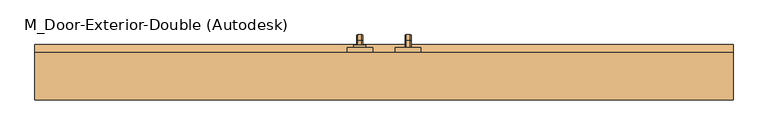
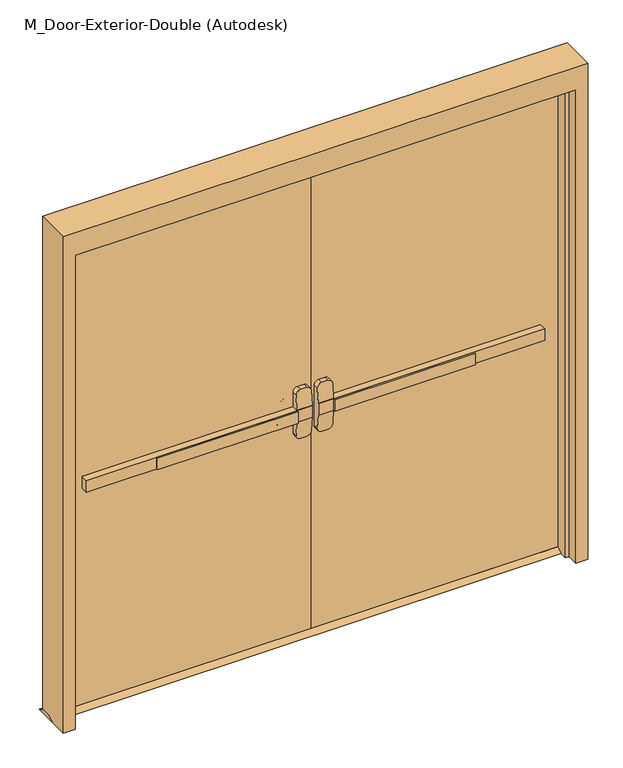
"""IFC4 building model written with IfcOpenShell, lengths in millimetres: door geometry, M_Door-Exterior-Double (Autodesk) : H_DR_AMD_Double Door_Ext_Steel_2100x2100_Panic Bar."""

from ifc_helpers import new_model, si_unit, point, frame, frame_2d, origin, place, context, project, spatial, polyline, circle_curve, ellipse_curve, trimmed, segment, composite_curve, outline, extrude, faceted_brep, source, transform, mapped, element, save
from ifc_brep_helpers import plane_surface, cylinder_surface, revolved_surface, advanced_brep


def m_door_exterior_double_autodesk_2b3cb0e1(model_context):
    return source(origin(), model_context, "Body", "SolidModel", [
        extrude(outline(polyline([(-666.1333333, -41.75), (-666.1333333, -35.4), (-76.2, -35.4), (-76.2, -41.75), (-666.1333333, -41.75)])), frame((0.0, 0.0, 974.6), z_axis=(0.0, 0.0, 1.0), x_axis=(1.0, 0.0, 0.0)), (0.0, 0.0, 1.0), 50.8),
        advanced_brep(
        [(-12.7, -35.4, 1025.4), (-76.2, -35.4, 1025.4), (-961.1, -35.4, 1025.4), (-961.1, -35.4, 974.6), (-76.2, -35.4, 974.6), (-12.7, -35.4, 974.6), (-961.1, -3.65, 1025.4), (-76.2, -3.65, 1025.4), (-76.2, -3.65, 1088.9), (-57.15, -3.65, 1107.95), (-31.75, -3.65, 1107.95), (-12.7, -3.65, 1088.9), (-12.7, -3.65, 911.1), (-31.75, -3.65, 892.05), (-57.15, -3.65, 892.05), (-76.2, -3.65, 911.1), (-76.2, -3.65, 974.6), (-961.1, -3.65, 974.6), (-12.7, -32.2247533, 1025.4), (-76.2, -32.2247533, 1025.4), (-12.7, -32.2247533, 974.6), (-12.7, -27.2145731, 911.1), (-12.7, -27.2145731, 1088.9), (-76.2, -32.2247533, 974.6), (-76.2, -27.2145731, 1088.9), (-76.2, -27.2145731, 911.1), (-57.15, -25.711519, 1107.95), (-31.75, -25.711519, 1107.95), (-31.75, -25.711519, 892.05), (-57.15, -25.711519, 892.05)],
        [
            (0, 1),
            (1, 2),
            (2, 3),
            (3, 4),
            (4, 5),
            (5, 0),
            (6, 7),
            (7, 8),
            (8, 9, circle_curve(frame((-57.15, -3.65, 1088.9), z_axis=(0.0, 1.0, 0.0), x_axis=(-1.0, 0.0, 0.0)), 19.05)),
            (9, 10),
            (10, 11, circle_curve(frame((-31.75, -3.65, 1088.9), z_axis=(0.0, 1.0, 0.0), x_axis=(-1.0, 0.0, 0.0)), 19.05)),
            (11, 12),
            (12, 13, circle_curve(frame((-31.75, -3.65, 911.1), z_axis=(0.0, 1.0, 0.0), x_axis=(-1.0, 0.0, 0.0)), 19.05)),
            (13, 14),
            (14, 15, circle_curve(frame((-57.15, -3.65, 911.1), z_axis=(0.0, 1.0, 0.0), x_axis=(-1.0, 0.0, 0.0)), 19.05)),
            (15, 16),
            (16, 17),
            (17, 6),
            (0, 18),
            (18, 19),
            (19, 7),
            (6, 2),
            (5, 20),
            (20, 21),
            (21, 12),
            (11, 22),
            (22, 18),
            (16, 23),
            (23, 20),
            (3, 17),
            (19, 24),
            (24, 8),
            (15, 25),
            (25, 23),
            (9, 26),
            (26, 27),
            (27, 10),
            (13, 28),
            (28, 29),
            (29, 14),
            (29, 25, ellipse_curve(frame((-57.15, -27.2145731, 911.1), z_axis=(0.0, 0.9969018152893365, 0.07865602756830282), x_axis=(0.0, -0.07865602756830208, 0.9969018152893365)), 19.1092038, 19.05)),
            (24, 26, ellipse_curve(frame((-57.15, -27.2145731, 1088.9), z_axis=(0.0, 0.9969018152893376, -0.07865602756828934), x_axis=(0.0, -0.078656027568288, -0.9969018152893377)), 19.1092038, 19.05)),
            (27, 22, ellipse_curve(frame((-31.75, -27.2145731, 1088.9), z_axis=(0.0, 0.9969018152893376, -0.07865602756828934), x_axis=(0.0, -0.078656027568288, -0.9969018152893377)), 19.1092038, 19.05)),
            (21, 28, ellipse_curve(frame((-31.75, -27.2145731, 911.1), z_axis=(0.0, 0.9969018152893365, 0.07865602756830282), x_axis=(0.0, -0.07865602756830208, 0.9969018152893365)), 19.1092038, 19.05)),
        ],
        [
            plane_surface(frame((-12.7, -35.4, 1025.4), z_axis=(0.0, -1.0, 0.0), x_axis=(1.0, 0.0, 0.0))),
            plane_surface(frame((-12.7, -3.65, 1025.4), z_axis=(0.0, 1.0, 0.0), x_axis=(-1.0, 0.0, 0.0))),
            plane_surface(frame((-961.1, -35.4, 1025.4), z_axis=(0.0, 0.0, 1.0), x_axis=(0.0, 1.0, 0.0))),
            plane_surface(frame((-12.7, -35.4, 1025.4), z_axis=(1.0, 0.0, 0.0), x_axis=(0.0, 1.0, 0.0))),
            plane_surface(frame((-12.7, -35.4, 974.6), z_axis=(0.0, 0.0, -1.0), x_axis=(0.0, 1.0, 0.0))),
            plane_surface(frame((-961.1, -35.4, 974.6), z_axis=(-1.0, 0.0, 0.0), x_axis=(0.0, 1.0, 0.0))),
            plane_surface(frame((-76.2, -32.2247533, 911.1), z_axis=(-1.0, 0.0, 0.0), x_axis=(0.0, 1.0, 0.0))),
            plane_surface(frame((-57.15, -32.2247533, 1107.95), z_axis=(0.0, 0.0, 1.0), x_axis=(0.0, 1.0, 0.0))),
            plane_surface(frame((-31.75, -32.2247533, 892.05), z_axis=(0.0, 0.0, -1.0), x_axis=(0.0, 1.0, 0.0))),
            cylinder_surface(frame((-57.15, -3.65, 911.1), z_axis=(0.0, -1.0, 0.0), x_axis=(-1.0, 0.0, 0.0)), 19.05),
            cylinder_surface(frame((-57.15, -3.65, 1088.9), z_axis=(0.0, -1.0, 0.0), x_axis=(-1.0, 0.0, 0.0)), 19.05),
            cylinder_surface(frame((-31.75, -3.65, 1088.9), z_axis=(0.0, -1.0, 0.0), x_axis=(-1.0, 0.0, 0.0)), 19.05),
            cylinder_surface(frame((-31.75, -3.65, 911.1), z_axis=(0.0, -1.0, 0.0), x_axis=(-1.0, 0.0, 0.0)), 19.05),
            plane_surface(frame((-76.2, -32.2247533, 1025.4), z_axis=(0.0, -0.9969018152893376, 0.07865602756828934), x_axis=(1.0, 0.0, 0.0))),
            plane_surface(frame((-76.2, -25.711519, 892.05), z_axis=(0.0, -0.9969018152893365, -0.07865602756830282), x_axis=(1.0, 0.0, 0.0))),
        ],
        [
            (0, [[1, 2, 3, 4, 5, 6]]),
            (1, [[7, 8, 9, 10, 11, 12, 13, 14, 15, 16, 17, 18]]),
            (2, [[-2, -1, 19, 20, 21, -7, 22]]),
            (3, [[23, 24, 25, -12, 26, 27, -19, -6]]),
            (4, [[-17, 28, 29, -23, -5, -4, 30]]),
            (5, [[-22, -18, -30, -3]]),
            (6, [[-21, 31, 32, -8]]),
            (6, [[33, 34, -28, -16]]),
            (7, [[35, 36, 37, -10]]),
            (8, [[38, 39, 40, -14]]),
            (9, [[-40, 41, -33, -15]]),
            (10, [[-32, 42, -35, -9]]),
            (11, [[-37, 43, -26, -11]]),
            (12, [[-25, 44, -38, -13]]),
            (13, [[-27, -43, -36, -42, -31, -20]]),
            (14, [[-29, -34, -41, -39, -44, -24]]),
        ],
    ),
        extrude(outline(polyline([(41.35, 15.0), (66.75, 0.0), (-29.05, 0.0), (-3.65, 15.0), (41.35, 15.0)])), frame((-1100.0, 0.0, 0.0), z_axis=(1.0, 0.0, 0.0), x_axis=(0.0, 1.0, 0.0)), (0.0, 0.0, 1.0), 2200.0),
        extrude(outline(polyline([(666.1333333, -41.75), (76.2, -41.75), (76.2, -35.4), (666.1333333, -35.4), (666.1333333, -41.75)])), frame((0.0, 0.0, 974.6), z_axis=(0.0, 0.0, 1.0), x_axis=(1.0, 0.0, 0.0)), (0.0, 0.0, 1.0), 50.8),
        advanced_brep(
        [(12.7, -35.4, 1025.4), (12.7, -35.4, 974.6), (76.2, -35.4, 974.6), (961.1, -35.4, 974.6), (961.1, -35.4, 1025.4), (76.2, -35.4, 1025.4), (961.1, -3.65, 1025.4), (961.1, -3.65, 974.6), (76.2, -3.65, 974.6), (76.2, -3.65, 911.1), (57.15, -3.65, 892.05), (31.75, -3.65, 892.05), (12.7, -3.65, 911.1), (12.7, -3.65, 1088.9), (31.75, -3.65, 1107.95), (57.15, -3.65, 1107.95), (76.2, -3.65, 1088.9), (76.2, -3.65, 1025.4), (76.2, -32.2247533, 1025.4), (12.7, -32.2247533, 1025.4), (12.7, -27.2145731, 1088.9), (12.7, -27.2145731, 911.1), (12.7, -32.2247533, 974.6), (76.2, -32.2247533, 974.6), (76.2, -27.2145731, 911.1), (76.2, -27.2145731, 1088.9), (31.75, -25.711519, 1107.95), (57.15, -25.711519, 1107.95), (57.15, -25.711519, 892.05), (31.75, -25.711519, 892.05)],
        [
            (0, 1),
            (1, 2),
            (2, 3),
            (3, 4),
            (4, 5),
            (5, 0),
            (6, 7),
            (7, 8),
            (8, 9),
            (9, 10, circle_curve(frame((57.15, -3.65, 911.1), z_axis=(0.0, 1.0, 0.0), x_axis=(1.0, 0.0, 0.0)), 19.05)),
            (10, 11),
            (11, 12, circle_curve(frame((31.75, -3.65, 911.1), z_axis=(0.0, 1.0, 0.0), x_axis=(1.0, 0.0, 0.0)), 19.05)),
            (12, 13),
            (13, 14, circle_curve(frame((31.75, -3.65, 1088.9), z_axis=(0.0, 1.0, 0.0), x_axis=(1.0, 0.0, 0.0)), 19.05)),
            (14, 15),
            (15, 16, circle_curve(frame((57.15, -3.65, 1088.9), z_axis=(0.0, 1.0, 0.0), x_axis=(1.0, 0.0, 0.0)), 19.05)),
            (16, 17),
            (17, 6),
            (4, 6),
            (17, 18),
            (18, 19),
            (19, 0),
            (19, 20),
            (20, 13),
            (12, 21),
            (21, 22),
            (22, 1),
            (7, 3),
            (22, 23),
            (23, 8),
            (23, 24),
            (24, 9),
            (16, 25),
            (25, 18),
            (14, 26),
            (26, 27),
            (27, 15),
            (10, 28),
            (28, 29),
            (29, 11),
            (24, 28, ellipse_curve(frame((57.15, -27.2145731, 911.1), z_axis=(0.0, 0.9969018152893365, 0.07865602756830282), x_axis=(0.0, -0.07865602756830208, 0.9969018152893365)), 19.1092038, 19.05)),
            (27, 25, ellipse_curve(frame((57.15, -27.2145731, 1088.9), z_axis=(0.0, 0.9969018152893376, -0.07865602756828934), x_axis=(0.0, -0.078656027568288, -0.9969018152893377)), 19.1092038, 19.05)),
            (20, 26, ellipse_curve(frame((31.75, -27.2145731, 1088.9), z_axis=(0.0, 0.9969018152893376, -0.07865602756828934), x_axis=(0.0, -0.078656027568288, -0.9969018152893377)), 19.1092038, 19.05)),
            (29, 21, ellipse_curve(frame((31.75, -27.2145731, 911.1), z_axis=(0.0, 0.9969018152893365, 0.07865602756830282), x_axis=(0.0, -0.07865602756830208, 0.9969018152893365)), 19.1092038, 19.05)),
        ],
        [
            plane_surface(frame((12.7, -35.4, 1025.4), z_axis=(0.0, -1.0, 0.0), x_axis=(-1.0, 0.0, 0.0))),
            plane_surface(frame((12.7, -3.65, 1025.4), z_axis=(0.0, 1.0, 0.0), x_axis=(1.0, 0.0, 0.0))),
            plane_surface(frame((961.1, -35.4, 1025.4), z_axis=(0.0, 0.0, 1.0), x_axis=(0.0, 1.0, 0.0))),
            plane_surface(frame((12.7, -35.4, 1025.4), z_axis=(-1.0, 0.0, 0.0), x_axis=(0.0, 1.0, 0.0))),
            plane_surface(frame((12.7, -35.4, 974.6), z_axis=(0.0, 0.0, -1.0), x_axis=(0.0, 1.0, 0.0))),
            plane_surface(frame((961.1, -35.4, 974.6), z_axis=(1.0, 0.0, 0.0), x_axis=(0.0, 1.0, 0.0))),
            plane_surface(frame((76.2, -32.2247533, 911.1), z_axis=(1.0, 0.0, 0.0), x_axis=(0.0, 1.0, 0.0))),
            plane_surface(frame((57.15, -32.2247533, 1107.95), z_axis=(0.0, 0.0, 1.0), x_axis=(0.0, 1.0, 0.0))),
            plane_surface(frame((31.75, -32.2247533, 892.05), z_axis=(0.0, 0.0, -1.0), x_axis=(0.0, 1.0, 0.0))),
            cylinder_surface(frame((57.15, -3.65, 911.1), z_axis=(0.0, -1.0, 0.0), x_axis=(1.0, 0.0, 0.0)), 19.05),
            cylinder_surface(frame((57.15, -3.65, 1088.9), z_axis=(0.0, -1.0, 0.0), x_axis=(1.0, 0.0, 0.0)), 19.05),
            cylinder_surface(frame((31.75, -3.65, 1088.9), z_axis=(0.0, -1.0, 0.0), x_axis=(1.0, 0.0, 0.0)), 19.05),
            cylinder_surface(frame((31.75, -3.65, 911.1), z_axis=(0.0, -1.0, 0.0), x_axis=(1.0, 0.0, 0.0)), 19.05),
            plane_surface(frame((76.2, -32.2247533, 1025.4), z_axis=(0.0, -0.9969018152893376, 0.07865602756828934), x_axis=(-1.0, 0.0, 0.0))),
            plane_surface(frame((76.2, -25.711519, 892.05), z_axis=(0.0, -0.9969018152893365, -0.07865602756830282), x_axis=(-1.0, 0.0, 0.0))),
        ],
        [
            (0, [[1, 2, 3, 4, 5, 6]]),
            (1, [[7, 8, 9, 10, 11, 12, 13, 14, 15, 16, 17, 18]]),
            (2, [[19, -18, 20, 21, 22, -6, -5]]),
            (3, [[-1, -22, 23, 24, -13, 25, 26, 27]]),
            (4, [[28, -3, -2, -27, 29, 30, -8]]),
            (5, [[-4, -28, -7, -19]]),
            (6, [[-9, -30, 31, 32]]),
            (6, [[-17, 33, 34, -20]]),
            (7, [[-15, 35, 36, 37]]),
            (8, [[-11, 38, 39, 40]]),
            (9, [[-10, -32, 41, -38]]),
            (10, [[-16, -37, 42, -33]]),
            (11, [[-14, -24, 43, -35]]),
            (12, [[-12, -40, 44, -25]]),
            (13, [[-21, -34, -42, -36, -43, -23]]),
            (14, [[-26, -44, -39, -41, -31, -29]]),
        ],
    ),
        advanced_brep(
        [(66.2, 54.05, 1001.190625), (66.2, 54.05, 998.809375), (69.771875, 54.05, 995.2375), (82.6284594, 54.05, 995.2375), (86.2, 54.05, 998.8090406), (86.2, 54.05, 1001.190625), (82.628125, 54.05, 1004.7625), (69.771875, 54.05, 1004.7625), (66.2, 54.05, 874.609375), (69.771875, 54.05, 871.0375), (82.628125, 54.05, 871.0375), (86.2, 54.05, 874.609375), (86.2, 54.05, 876.9909594), (82.6284594, 54.05, 880.5625), (69.771875, 54.05, 880.5625), (66.2, 54.05, 876.990625), (66.2, 79.45, 1001.190625), (66.2, 93.340625, 987.3), (66.2, 93.340625, 888.5), (66.2, 79.45, 874.609375), (66.2, 79.45, 876.990625), (66.2, 90.959375, 888.5), (66.2, 90.959375, 987.3), (66.2, 79.45, 998.809375), (69.771875, 79.45, 995.2375), (82.6284594, 79.45, 995.2375), (86.2, 79.45, 998.8090406), (86.2, 90.9590406, 987.3), (86.2, 90.9590406, 888.5), (86.2, 79.45, 876.9909594), (86.2, 79.45, 874.609375), (86.2, 93.340625, 888.5), (86.2, 93.340625, 987.3), (86.2, 79.45, 1001.190625), (82.628125, 79.45, 1004.7625), (69.771875, 79.45, 1004.7625), (69.771875, 87.3875, 987.3), (82.6284594, 87.3875, 987.3), (82.628125, 96.9125, 987.3), (69.771875, 96.9125, 987.3), (69.771875, 87.3875, 888.5), (82.6284594, 87.3875, 888.5), (82.628125, 96.9125, 888.5), (69.771875, 96.9125, 888.5), (69.771875, 79.45, 880.5625), (82.6284594, 79.45, 880.5625), (82.628125, 79.45, 871.0375), (69.771875, 79.45, 871.0375)],
        [
            (0, 1),
            (1, 2, circle_curve(frame((69.771875, 54.05, 998.809375), z_axis=(0.0, -1.0, 0.0), x_axis=(0.0, 0.0, 1.0)), 3.571875)),
            (2, 3),
            (3, 4, circle_curve(frame((82.6284594, 54.05, 998.8090406), z_axis=(0.0, -1.0, 0.0), x_axis=(0.0, 0.0, 1.0)), 3.5715406)),
            (4, 5),
            (5, 6, circle_curve(frame((82.628125, 54.05, 1001.190625), z_axis=(0.0, -1.0, 0.0), x_axis=(0.0, 0.0, 1.0)), 3.571875)),
            (6, 7),
            (7, 0, circle_curve(frame((69.771875, 54.05, 1001.190625), z_axis=(0.0, -1.0, 0.0), x_axis=(0.0, 0.0, 1.0)), 3.571875)),
            (8, 9, circle_curve(frame((69.771875, 54.05, 874.609375), z_axis=(0.0, -1.0, 0.0), x_axis=(0.0, 0.0, -1.0)), 3.571875)),
            (9, 10),
            (10, 11, circle_curve(frame((82.628125, 54.05, 874.609375), z_axis=(0.0, -1.0, 0.0), x_axis=(0.0, 0.0, -1.0)), 3.571875)),
            (11, 12),
            (12, 13, circle_curve(frame((82.6284594, 54.05, 876.9909594), z_axis=(0.0, -1.0, 0.0), x_axis=(0.0, 0.0, -1.0)), 3.5715406)),
            (13, 14),
            (14, 15, circle_curve(frame((69.771875, 54.05, 876.990625), z_axis=(0.0, -1.0, 0.0), x_axis=(0.0, 0.0, -1.0)), 3.571875)),
            (15, 8),
            (0, 16),
            (16, 17, circle_curve(frame((66.2, 79.45, 987.3), z_axis=(-1.0, 0.0, 0.0), x_axis=(0.0, 0.0, 1.0)), 13.890625)),
            (17, 18),
            (18, 19, circle_curve(frame((66.2, 79.45, 888.5), z_axis=(-1.0, 0.0, 0.0), x_axis=(0.0, 1.0, 0.0)), 13.890625)),
            (19, 8),
            (15, 20),
            (20, 21, circle_curve(frame((66.2, 79.45, 888.5), z_axis=(1.0, 0.0, 0.0), x_axis=(0.0, 1.0, 0.0)), 11.509375)),
            (21, 22),
            (22, 23, circle_curve(frame((66.2, 79.45, 987.3), z_axis=(1.0, 0.0, 0.0), x_axis=(0.0, 0.0, 1.0)), 11.509375)),
            (23, 1),
            (23, 24, circle_curve(frame((69.771875, 79.45, 998.809375), z_axis=(0.0, -1.0, 0.0), x_axis=(0.0, 0.0, 1.0)), 3.571875)),
            (24, 2),
            (24, 25),
            (25, 3),
            (25, 26, circle_curve(frame((82.6284594, 79.45, 998.8090406), z_axis=(0.0, -1.0, 0.0), x_axis=(0.0, 0.0, 1.0)), 3.5715406)),
            (26, 4),
            (26, 27, circle_curve(frame((86.2, 79.45, 987.3), z_axis=(-1.0, 0.0, 0.0), x_axis=(0.0, 0.0, 1.0)), 11.5090406)),
            (27, 28),
            (28, 29, circle_curve(frame((86.2, 79.45, 888.5), z_axis=(-1.0, 0.0, 0.0), x_axis=(0.0, 1.0, 0.0)), 11.5090406)),
            (29, 12),
            (11, 30),
            (30, 31, circle_curve(frame((86.2, 79.45, 888.5), z_axis=(1.0, 0.0, 0.0), x_axis=(0.0, 1.0, 0.0)), 13.890625)),
            (31, 32),
            (32, 33, circle_curve(frame((86.2, 79.45, 987.3), z_axis=(1.0, 0.0, 0.0), x_axis=(0.0, 0.0, 1.0)), 13.890625)),
            (33, 5),
            (33, 34, circle_curve(frame((82.628125, 79.45, 1001.190625), z_axis=(0.0, -1.0, 0.0), x_axis=(0.0, 0.0, 1.0)), 3.571875)),
            (34, 6),
            (34, 35),
            (35, 7),
            (35, 16, circle_curve(frame((69.771875, 79.45, 1001.190625), z_axis=(0.0, -1.0, 0.0), x_axis=(0.0, 0.0, 1.0)), 3.571875)),
            (36, 24, circle_curve(frame((69.771875, 79.45, 987.3), z_axis=(1.0, 0.0, 0.0), x_axis=(0.0, 0.0, 1.0)), 7.9375)),
            (22, 36, circle_curve(frame((69.771875, 90.959375, 987.3), z_axis=(0.0, 0.0, 1.0), x_axis=(0.0, 1.0, 0.0)), 3.571875)),
            (37, 25, circle_curve(frame((82.6284594, 79.45, 987.3), z_axis=(1.0, 0.0, 0.0), x_axis=(0.0, 0.0, 1.0)), 7.9375)),
            (36, 37),
            (37, 27, circle_curve(frame((82.6284594, 90.9590406, 987.3), z_axis=(0.0, 0.0, 1.0), x_axis=(0.0, 1.0, 0.0)), 3.5715406)),
            (38, 34, circle_curve(frame((82.628125, 79.45, 987.3), z_axis=(1.0, 0.0, 0.0), x_axis=(0.0, 0.0, 1.0)), 17.4625)),
            (32, 38, circle_curve(frame((82.628125, 93.340625, 987.3), z_axis=(0.0, 0.0, 1.0), x_axis=(0.0, 1.0, 0.0)), 3.571875)),
            (39, 35, circle_curve(frame((69.771875, 79.45, 987.3), z_axis=(1.0, 0.0, 0.0), x_axis=(0.0, 0.0, 1.0)), 17.4625)),
            (38, 39),
            (39, 17, circle_curve(frame((69.771875, 93.340625, 987.3), z_axis=(0.0, 0.0, 1.0), x_axis=(0.0, 1.0, 0.0)), 3.571875)),
            (21, 40, circle_curve(frame((69.771875, 90.959375, 888.5), z_axis=(0.0, 0.0, 1.0), x_axis=(0.0, 1.0, 0.0)), 3.571875)),
            (40, 36),
            (40, 41),
            (41, 37),
            (41, 28, circle_curve(frame((82.6284594, 90.9590406, 888.5), z_axis=(0.0, 0.0, 1.0), x_axis=(0.0, 1.0, 0.0)), 3.5715406)),
            (31, 42, circle_curve(frame((82.628125, 93.340625, 888.5), z_axis=(0.0, 0.0, 1.0), x_axis=(0.0, 1.0, 0.0)), 3.571875)),
            (42, 38),
            (42, 43),
            (43, 39),
            (43, 18, circle_curve(frame((69.771875, 93.340625, 888.5), z_axis=(0.0, 0.0, 1.0), x_axis=(0.0, 1.0, 0.0)), 3.571875)),
            (44, 40, circle_curve(frame((69.771875, 79.45, 888.5), z_axis=(1.0, 0.0, 0.0), x_axis=(0.0, 1.0, 0.0)), 7.9375)),
            (20, 44, circle_curve(frame((69.771875, 79.45, 876.990625), z_axis=(0.0, 1.0, 0.0), x_axis=(0.0, 0.0, -1.0)), 3.571875)),
            (45, 41, circle_curve(frame((82.6284594, 79.45, 888.5), z_axis=(1.0, 0.0, 0.0), x_axis=(0.0, 1.0, 0.0)), 7.9375)),
            (44, 45),
            (45, 29, circle_curve(frame((82.6284594, 79.45, 876.9909594), z_axis=(0.0, 1.0, 0.0), x_axis=(0.0, 0.0, -1.0)), 3.5715406)),
            (46, 42, circle_curve(frame((82.628125, 79.45, 888.5), z_axis=(1.0, 0.0, 0.0), x_axis=(0.0, 1.0, 0.0)), 17.4625)),
            (30, 46, circle_curve(frame((82.628125, 79.45, 874.609375), z_axis=(0.0, 1.0, 0.0), x_axis=(0.0, 0.0, -1.0)), 3.571875)),
            (47, 43, circle_curve(frame((69.771875, 79.45, 888.5), z_axis=(1.0, 0.0, 0.0), x_axis=(0.0, 1.0, 0.0)), 17.4625)),
            (46, 47),
            (47, 19, circle_curve(frame((69.771875, 79.45, 874.609375), z_axis=(0.0, 1.0, 0.0), x_axis=(0.0, 0.0, -1.0)), 3.571875)),
            (14, 44),
            (13, 45),
            (10, 46),
            (9, 47),
        ],
        [
            plane_surface(frame((76.2, 54.05, 1000.0), z_axis=(0.0, -1.0, 0.0), x_axis=(1.0, 0.0, 0.0))),
            plane_surface(frame((76.2, 54.05, 875.8), z_axis=(0.0, -1.0, 0.0), x_axis=(1.0, 0.0, 0.0))),
            plane_surface(frame((66.2, 54.05, 1001.190625), z_axis=(-1.0, 0.0, 0.0), x_axis=(0.0, 1.0, 0.0))),
            cylinder_surface(frame((69.771875, 54.05, 998.809375), z_axis=(0.0, -1.0, 0.0), x_axis=(0.0, 0.0, 1.0)), 3.571875),
            plane_surface(frame((69.771875, 54.05, 995.2375), z_axis=(0.0, 0.0, -1.0), x_axis=(0.0, 1.0, 0.0))),
            cylinder_surface(frame((82.6284594, 54.05, 998.8090406), z_axis=(0.0, -1.0, 0.0), x_axis=(0.0, 0.0, 1.0)), 3.5715406),
            plane_surface(frame((86.2, 54.05, 998.8090406), z_axis=(1.0, 0.0, 0.0), x_axis=(0.0, 1.0, 0.0))),
            cylinder_surface(frame((82.628125, 54.05, 1001.190625), z_axis=(0.0, -1.0, 0.0), x_axis=(0.0, 0.0, 1.0)), 3.571875),
            plane_surface(frame((82.628125, 54.05, 1004.7625), z_axis=(0.0, 0.0, 1.0), x_axis=(0.0, 1.0, 0.0))),
            cylinder_surface(frame((69.771875, 54.05, 1001.190625), z_axis=(0.0, -1.0, 0.0), x_axis=(0.0, 0.0, 1.0)), 3.571875),
            revolved_surface(trimmed(ellipse_curve(frame((69.771875, 79.45, 998.809375), z_axis=(0.0, -1.0, 0.0), x_axis=(0.0, 0.0, 1.0)), 3.571875, 3.571875), [point((66.2, 79.45, 998.809375))], [point((69.771875, 79.45, 995.2375))], True, "CARTESIAN"), (76.2, 79.45, 987.3), (-1.0, 0.0, 0.0)),
            revolved_surface(polyline([(69.771875, 79.45, 995.2375), (82.6284594, 79.45, 995.2375)]), (76.2, 79.45, 987.3), (-1.0, 0.0, 0.0)),
            revolved_surface(trimmed(ellipse_curve(frame((82.6284594, 79.45, 998.8090406), z_axis=(0.0, -1.0, 0.0), x_axis=(0.0, 0.0, 1.0)), 3.5715406, 3.5715406), [point((82.6284594, 79.45, 995.2375))], [point((86.2, 79.45, 998.8090406))], True, "CARTESIAN"), (76.2, 79.45, 987.3), (-1.0, 0.0, 0.0)),
            revolved_surface(trimmed(ellipse_curve(frame((82.628125, 79.45, 1001.190625), z_axis=(0.0, -1.0, 0.0), x_axis=(0.0, 0.0, 1.0)), 3.571875, 3.571875), [point((86.2, 79.45, 1001.190625))], [point((82.628125, 79.45, 1004.7625))], True, "CARTESIAN"), (76.2, 79.45, 987.3), (-1.0, 0.0, 0.0)),
            cylinder_surface(frame((76.2, 79.45, 987.3), z_axis=(-1.0, 0.0, 0.0), x_axis=(0.0, 0.0, 1.0)), 17.4625),
            revolved_surface(trimmed(ellipse_curve(frame((69.771875, 79.45, 1001.190625), z_axis=(0.0, -1.0, 0.0), x_axis=(0.0, 0.0, 1.0)), 3.571875, 3.571875), [point((69.771875, 79.45, 1004.7625))], [point((66.2, 79.45, 1001.190625))], True, "CARTESIAN"), (76.2, 79.45, 987.3), (-1.0, 0.0, 0.0)),
            cylinder_surface(frame((69.771875, 90.959375, 987.3), z_axis=(0.0, 0.0, 1.0), x_axis=(0.0, 1.0, 0.0)), 3.571875),
            plane_surface(frame((69.771875, 87.3875, 987.3), z_axis=(0.0, -1.0, 0.0), x_axis=(0.0, 0.0, -1.0))),
            cylinder_surface(frame((82.6284594, 90.9590406, 987.3), z_axis=(0.0, 0.0, 1.0), x_axis=(0.0, 1.0, 0.0)), 3.5715406),
            cylinder_surface(frame((82.628125, 93.340625, 987.3), z_axis=(0.0, 0.0, 1.0), x_axis=(0.0, 1.0, 0.0)), 3.571875),
            plane_surface(frame((82.628125, 96.9125, 987.3), z_axis=(0.0, 1.0, 0.0), x_axis=(0.0, 0.0, -1.0))),
            cylinder_surface(frame((69.771875, 93.340625, 987.3), z_axis=(0.0, 0.0, 1.0), x_axis=(0.0, 1.0, 0.0)), 3.571875),
            revolved_surface(trimmed(ellipse_curve(frame((69.771875, 90.959375, 888.5), z_axis=(0.0, 0.0, 1.0), x_axis=(0.0, 1.0, 0.0)), 3.571875, 3.571875), [point((66.2, 90.959375, 888.5))], [point((69.771875, 87.3875, 888.5))], True, "CARTESIAN"), (76.2, 79.45, 888.5), (-1.0, 0.0, 0.0)),
            revolved_surface(polyline([(69.771875, 87.3875, 888.5), (82.6284594, 87.3875, 888.5)]), (76.2, 79.45, 888.5), (-1.0, 0.0, 0.0)),
            revolved_surface(trimmed(ellipse_curve(frame((82.6284594, 90.9590406, 888.5), z_axis=(0.0, 0.0, 1.0), x_axis=(0.0, 1.0, 0.0)), 3.5715406, 3.5715406), [point((82.6284594, 87.3875, 888.5))], [point((86.2, 90.9590406, 888.5))], True, "CARTESIAN"), (76.2, 79.45, 888.5), (-1.0, 0.0, 0.0)),
            revolved_surface(trimmed(ellipse_curve(frame((82.628125, 93.340625, 888.5), z_axis=(0.0, 0.0, 1.0), x_axis=(0.0, 1.0, 0.0)), 3.571875, 3.571875), [point((86.2, 93.340625, 888.5))], [point((82.628125, 96.9125, 888.5))], True, "CARTESIAN"), (76.2, 79.45, 888.5), (-1.0, 0.0, 0.0)),
            cylinder_surface(frame((76.2, 79.45, 888.5), z_axis=(-1.0, 0.0, 0.0), x_axis=(0.0, 1.0, 0.0)), 17.4625),
            revolved_surface(trimmed(ellipse_curve(frame((69.771875, 93.340625, 888.5), z_axis=(0.0, 0.0, 1.0), x_axis=(0.0, 1.0, 0.0)), 3.571875, 3.571875), [point((69.771875, 96.9125, 888.5))], [point((66.2, 93.340625, 888.5))], True, "CARTESIAN"), (76.2, 79.45, 888.5), (-1.0, 0.0, 0.0)),
            cylinder_surface(frame((69.771875, 79.45, 876.990625), z_axis=(0.0, 1.0, 0.0), x_axis=(0.0, 0.0, -1.0)), 3.571875),
            plane_surface(frame((69.771875, 79.45, 880.5625), z_axis=(0.0, 0.0, 1.0), x_axis=(0.0, -1.0, 0.0))),
            cylinder_surface(frame((82.6284594, 79.45, 876.9909594), z_axis=(0.0, 1.0, 0.0), x_axis=(0.0, 0.0, -1.0)), 3.5715406),
            cylinder_surface(frame((82.628125, 79.45, 874.609375), z_axis=(0.0, 1.0, 0.0), x_axis=(0.0, 0.0, -1.0)), 3.571875),
            plane_surface(frame((82.628125, 79.45, 871.0375), z_axis=(0.0, 0.0, -1.0), x_axis=(0.0, -1.0, 0.0))),
            cylinder_surface(frame((69.771875, 79.45, 874.609375), z_axis=(0.0, 1.0, 0.0), x_axis=(0.0, 0.0, -1.0)), 3.571875),
        ],
        [
            (0, [[1, 2, 3, 4, 5, 6, 7, 8]]),
            (1, [[9, 10, 11, 12, 13, 14, 15, 16]]),
            (2, [[-1, 17, 18, 19, 20, 21, -16, 22, 23, 24, 25, 26]]),
            (3, [[-2, -26, 27, 28]]),
            (4, [[-3, -28, 29, 30]]),
            (5, [[-4, -30, 31, 32]]),
            (6, [[-5, -32, 33, 34, 35, 36, -12, 37, 38, 39, 40, 41]]),
            (7, [[-6, -41, 42, 43]]),
            (8, [[-7, -43, 44, 45]]),
            (9, [[-8, -45, 46, -17]]),
            (10, [[47, -27, -25, 48]]),
            (11, [[49, -29, -47, 50]]),
            (12, [[-33, -31, -49, 51]]),
            (13, [[52, -42, -40, 53]]),
            (14, [[54, -44, -52, 55]]),
            (15, [[-18, -46, -54, 56]]),
            (16, [[-48, -24, 57, 58]]),
            (17, [[-50, -58, 59, 60]]),
            (18, [[-51, -60, 61, -34]]),
            (19, [[-53, -39, 62, 63]]),
            (20, [[-55, -63, 64, 65]]),
            (21, [[-56, -65, 66, -19]]),
            (22, [[67, -57, -23, 68]]),
            (23, [[69, -59, -67, 70]]),
            (24, [[-35, -61, -69, 71]]),
            (25, [[72, -62, -38, 73]]),
            (26, [[74, -64, -72, 75]]),
            (27, [[-20, -66, -74, 76]]),
            (28, [[-68, -22, -15, 77]]),
            (29, [[-70, -77, -14, 78]]),
            (30, [[-71, -78, -13, -36]]),
            (31, [[-73, -37, -11, 79]]),
            (32, [[-75, -79, -10, 80]]),
            (33, [[-76, -80, -9, -21]]),
        ],
    ),
        extrude(outline(composite_curve([segment(trimmed(circle_curve(frame_2d((1094.2338574, 76.2)), 90.1286291), [point((1175.0, 116.2))], [point((1175.0, 36.2))], False, "CARTESIAN"), True, "CONTINUOUS"), segment(polyline([(1175.0, 36.2), (825.0, 36.2)]), True, "CONTINUOUS"), segment(trimmed(circle_curve(frame_2d((905.7661426, 76.2)), 90.1286291), [point((825.0, 36.2))], [point((825.0, 116.2))], False, "CARTESIAN"), True, "CONTINUOUS"), segment(polyline([(825.0, 116.2), (1175.0, 116.2)]), True, "CONTINUOUS")], self_intersect=False)), frame((0.0, 41.35, 0.0), z_axis=(0.0, 1.0, 0.0), x_axis=(0.0, 0.0, 1.0)), (0.0, 0.0, 1.0), 15.0),
        advanced_brep(
        [(-86.2, 54.05, 1001.190625), (-86.2, 54.05, 998.809375), (-82.628125, 54.05, 995.2375), (-69.7715406, 54.05, 995.2375), (-66.2, 54.05, 998.8090406), (-66.2, 54.05, 1001.190625), (-69.771875, 54.05, 1004.7625), (-82.628125, 54.05, 1004.7625), (-86.2, 54.05, 874.609375), (-82.628125, 54.05, 871.0375), (-69.771875, 54.05, 871.0375), (-66.2, 54.05, 874.609375), (-66.2, 54.05, 876.9909594), (-69.7715406, 54.05, 880.5625), (-82.628125, 54.05, 880.5625), (-86.2, 54.05, 876.990625), (-86.2, 79.45, 1001.190625), (-86.2, 93.340625, 987.3), (-86.2, 93.340625, 888.5), (-86.2, 79.45, 874.609375), (-86.2, 79.45, 876.990625), (-86.2, 90.959375, 888.5), (-86.2, 90.959375, 987.3), (-86.2, 79.45, 998.809375), (-82.628125, 79.45, 995.2375), (-69.7715406, 79.45, 995.2375), (-66.2, 79.45, 998.8090406), (-66.2, 90.9590406, 987.3), (-66.2, 90.9590406, 888.5), (-66.2, 79.45, 876.9909594), (-66.2, 79.45, 874.609375), (-66.2, 93.340625, 888.5), (-66.2, 93.340625, 987.3), (-66.2, 79.45, 1001.190625), (-69.771875, 79.45, 1004.7625), (-82.628125, 79.45, 1004.7625), (-82.628125, 87.3875, 987.3), (-69.7715406, 87.3875, 987.3), (-69.771875, 96.9125, 987.3), (-82.628125, 96.9125, 987.3), (-82.628125, 87.3875, 888.5), (-69.7715406, 87.3875, 888.5), (-69.771875, 96.9125, 888.5), (-82.628125, 96.9125, 888.5), (-82.628125, 79.45, 880.5625), (-69.7715406, 79.45, 880.5625), (-69.771875, 79.45, 871.0375), (-82.628125, 79.45, 871.0375)],
        [
            (0, 1),
            (1, 2, circle_curve(frame((-82.628125, 54.05, 998.809375), z_axis=(0.0, -1.0, 0.0), x_axis=(0.0, 0.0, 1.0)), 3.571875)),
            (2, 3),
            (3, 4, circle_curve(frame((-69.7715406, 54.05, 998.8090406), z_axis=(0.0, -1.0, 0.0), x_axis=(0.0, 0.0, 1.0)), 3.5715406)),
            (4, 5),
            (5, 6, circle_curve(frame((-69.771875, 54.05, 1001.190625), z_axis=(0.0, -1.0, 0.0), x_axis=(0.0, 0.0, 1.0)), 3.571875)),
            (6, 7),
            (7, 0, circle_curve(frame((-82.628125, 54.05, 1001.190625), z_axis=(0.0, -1.0, 0.0), x_axis=(0.0, 0.0, 1.0)), 3.571875)),
            (8, 9, circle_curve(frame((-82.628125, 54.05, 874.609375), z_axis=(0.0, -1.0, 0.0), x_axis=(0.0, 0.0, -1.0)), 3.571875)),
            (9, 10),
            (10, 11, circle_curve(frame((-69.771875, 54.05, 874.609375), z_axis=(0.0, -1.0, 0.0), x_axis=(0.0, 0.0, -1.0)), 3.571875)),
            (11, 12),
            (12, 13, circle_curve(frame((-69.7715406, 54.05, 876.9909594), z_axis=(0.0, -1.0, 0.0), x_axis=(0.0, 0.0, -1.0)), 3.5715406)),
            (13, 14),
            (14, 15, circle_curve(frame((-82.628125, 54.05, 876.990625), z_axis=(0.0, -1.0, 0.0), x_axis=(0.0, 0.0, -1.0)), 3.571875)),
            (15, 8),
            (0, 16),
            (16, 17, circle_curve(frame((-86.2, 79.45, 987.3), z_axis=(-1.0, 0.0, 0.0), x_axis=(0.0, 0.0, 1.0)), 13.890625)),
            (17, 18),
            (18, 19, circle_curve(frame((-86.2, 79.45, 888.5), z_axis=(-1.0, 0.0, 0.0), x_axis=(0.0, 1.0, 0.0)), 13.890625)),
            (19, 8),
            (15, 20),
            (20, 21, circle_curve(frame((-86.2, 79.45, 888.5), z_axis=(1.0, 0.0, 0.0), x_axis=(0.0, 1.0, 0.0)), 11.509375)),
            (21, 22),
            (22, 23, circle_curve(frame((-86.2, 79.45, 987.3), z_axis=(1.0, 0.0, 0.0), x_axis=(0.0, 0.0, 1.0)), 11.509375)),
            (23, 1),
            (23, 24, circle_curve(frame((-82.628125, 79.45, 998.809375), z_axis=(0.0, -1.0, 0.0), x_axis=(0.0, 0.0, 1.0)), 3.571875)),
            (24, 2),
            (24, 25),
            (25, 3),
            (25, 26, circle_curve(frame((-69.7715406, 79.45, 998.8090406), z_axis=(0.0, -1.0, 0.0), x_axis=(0.0, 0.0, 1.0)), 3.5715406)),
            (26, 4),
            (26, 27, circle_curve(frame((-66.2, 79.45, 987.3), z_axis=(-1.0, 0.0, 0.0), x_axis=(0.0, 0.0, 1.0)), 11.5090406)),
            (27, 28),
            (28, 29, circle_curve(frame((-66.2, 79.45, 888.5), z_axis=(-1.0, 0.0, 0.0), x_axis=(0.0, 1.0, 0.0)), 11.5090406)),
            (29, 12),
            (11, 30),
            (30, 31, circle_curve(frame((-66.2, 79.45, 888.5), z_axis=(1.0, 0.0, 0.0), x_axis=(0.0, 1.0, 0.0)), 13.890625)),
            (31, 32),
            (32, 33, circle_curve(frame((-66.2, 79.45, 987.3), z_axis=(1.0, 0.0, 0.0), x_axis=(0.0, 0.0, 1.0)), 13.890625)),
            (33, 5),
            (33, 34, circle_curve(frame((-69.771875, 79.45, 1001.190625), z_axis=(0.0, -1.0, 0.0), x_axis=(0.0, 0.0, 1.0)), 3.571875)),
            (34, 6),
            (34, 35),
            (35, 7),
            (35, 16, circle_curve(frame((-82.628125, 79.45, 1001.190625), z_axis=(0.0, -1.0, 0.0), x_axis=(0.0, 0.0, 1.0)), 3.571875)),
            (36, 24, circle_curve(frame((-82.628125, 79.45, 987.3), z_axis=(1.0, 0.0, 0.0), x_axis=(0.0, 0.0, 1.0)), 7.9375)),
            (22, 36, circle_curve(frame((-82.628125, 90.959375, 987.3), z_axis=(0.0, 0.0, 1.0), x_axis=(0.0, 1.0, 0.0)), 3.571875)),
            (37, 25, circle_curve(frame((-69.7715406, 79.45, 987.3), z_axis=(1.0, 0.0, 0.0), x_axis=(0.0, 0.0, 1.0)), 7.9375)),
            (36, 37),
            (37, 27, circle_curve(frame((-69.7715406, 90.9590406, 987.3), z_axis=(0.0, 0.0, 1.0), x_axis=(0.0, 1.0, 0.0)), 3.5715406)),
            (38, 34, circle_curve(frame((-69.771875, 79.45, 987.3), z_axis=(1.0, 0.0, 0.0), x_axis=(0.0, 0.0, 1.0)), 17.4625)),
            (32, 38, circle_curve(frame((-69.771875, 93.340625, 987.3), z_axis=(0.0, 0.0, 1.0), x_axis=(0.0, 1.0, 0.0)), 3.571875)),
            (39, 35, circle_curve(frame((-82.628125, 79.45, 987.3), z_axis=(1.0, 0.0, 0.0), x_axis=(0.0, 0.0, 1.0)), 17.4625)),
            (38, 39),
            (39, 17, circle_curve(frame((-82.628125, 93.340625, 987.3), z_axis=(0.0, 0.0, 1.0), x_axis=(0.0, 1.0, 0.0)), 3.571875)),
            (21, 40, circle_curve(frame((-82.628125, 90.959375, 888.5), z_axis=(0.0, 0.0, 1.0), x_axis=(0.0, 1.0, 0.0)), 3.571875)),
            (40, 36),
            (40, 41),
            (41, 37),
            (41, 28, circle_curve(frame((-69.7715406, 90.9590406, 888.5), z_axis=(0.0, 0.0, 1.0), x_axis=(0.0, 1.0, 0.0)), 3.5715406)),
            (31, 42, circle_curve(frame((-69.771875, 93.340625, 888.5), z_axis=(0.0, 0.0, 1.0), x_axis=(0.0, 1.0, 0.0)), 3.571875)),
            (42, 38),
            (42, 43),
            (43, 39),
            (43, 18, circle_curve(frame((-82.628125, 93.340625, 888.5), z_axis=(0.0, 0.0, 1.0), x_axis=(0.0, 1.0, 0.0)), 3.571875)),
            (44, 40, circle_curve(frame((-82.628125, 79.45, 888.5), z_axis=(1.0, 0.0, 0.0), x_axis=(0.0, 1.0, 0.0)), 7.9375)),
            (20, 44, circle_curve(frame((-82.628125, 79.45, 876.990625), z_axis=(0.0, 1.0, 0.0), x_axis=(0.0, 0.0, -1.0)), 3.571875)),
            (45, 41, circle_curve(frame((-69.7715406, 79.45, 888.5), z_axis=(1.0, 0.0, 0.0), x_axis=(0.0, 1.0, 0.0)), 7.9375)),
            (44, 45),
            (45, 29, circle_curve(frame((-69.7715406, 79.45, 876.9909594), z_axis=(0.0, 1.0, 0.0), x_axis=(0.0, 0.0, -1.0)), 3.5715406)),
            (46, 42, circle_curve(frame((-69.771875, 79.45, 888.5), z_axis=(1.0, 0.0, 0.0), x_axis=(0.0, 1.0, 0.0)), 17.4625)),
            (30, 46, circle_curve(frame((-69.771875, 79.45, 874.609375), z_axis=(0.0, 1.0, 0.0), x_axis=(0.0, 0.0, -1.0)), 3.571875)),
            (47, 43, circle_curve(frame((-82.628125, 79.45, 888.5), z_axis=(1.0, 0.0, 0.0), x_axis=(0.0, 1.0, 0.0)), 17.4625)),
            (46, 47),
            (47, 19, circle_curve(frame((-82.628125, 79.45, 874.609375), z_axis=(0.0, 1.0, 0.0), x_axis=(0.0, 0.0, -1.0)), 3.571875)),
            (14, 44),
            (13, 45),
            (10, 46),
            (9, 47),
        ],
        [
            plane_surface(frame((-76.2, 54.05, 1000.0), z_axis=(0.0, -1.0, 0.0), x_axis=(1.0, 0.0, 0.0))),
            plane_surface(frame((-76.2, 54.05, 875.8), z_axis=(0.0, -1.0, 0.0), x_axis=(1.0, 0.0, 0.0))),
            plane_surface(frame((-86.2, 54.05, 1001.190625), z_axis=(-1.0, 0.0, 0.0), x_axis=(0.0, 1.0, 0.0))),
            cylinder_surface(frame((-82.628125, 54.05, 998.809375), z_axis=(0.0, -1.0, 0.0), x_axis=(0.0, 0.0, 1.0)), 3.571875),
            plane_surface(frame((-82.628125, 54.05, 995.2375), z_axis=(0.0, 0.0, -1.0), x_axis=(0.0, 1.0, 0.0))),
            cylinder_surface(frame((-69.7715406, 54.05, 998.8090406), z_axis=(0.0, -1.0, 0.0), x_axis=(0.0, 0.0, 1.0)), 3.5715406),
            plane_surface(frame((-66.2, 54.05, 998.8090406), z_axis=(1.0, 0.0, 0.0), x_axis=(0.0, 1.0, 0.0))),
            cylinder_surface(frame((-69.771875, 54.05, 1001.190625), z_axis=(0.0, -1.0, 0.0), x_axis=(0.0, 0.0, 1.0)), 3.571875),
            plane_surface(frame((-69.771875, 54.05, 1004.7625), z_axis=(0.0, 0.0, 1.0), x_axis=(0.0, 1.0, 0.0))),
            cylinder_surface(frame((-82.628125, 54.05, 1001.190625), z_axis=(0.0, -1.0, 0.0), x_axis=(0.0, 0.0, 1.0)), 3.571875),
            revolved_surface(trimmed(ellipse_curve(frame((-82.628125, 79.45, 998.809375), z_axis=(0.0, -1.0, 0.0), x_axis=(0.0, 0.0, 1.0)), 3.571875, 3.571875), [point((-86.2, 79.45, 998.809375))], [point((-82.628125, 79.45, 995.2375))], True, "CARTESIAN"), (-76.2, 79.45, 987.3), (-1.0, 0.0, 0.0)),
            revolved_surface(polyline([(-82.628125, 79.45, 995.2375), (-69.7715406, 79.45, 995.2375)]), (-76.2, 79.45, 987.3), (-1.0, 0.0, 0.0)),
            revolved_surface(trimmed(ellipse_curve(frame((-69.7715406, 79.45, 998.8090406), z_axis=(0.0, -1.0, 0.0), x_axis=(0.0, 0.0, 1.0)), 3.5715406, 3.5715406), [point((-69.7715406, 79.45, 995.2375))], [point((-66.2, 79.45, 998.8090406))], True, "CARTESIAN"), (-76.2, 79.45, 987.3), (-1.0, 0.0, 0.0)),
            revolved_surface(trimmed(ellipse_curve(frame((-69.771875, 79.45, 1001.190625), z_axis=(0.0, -1.0, 0.0), x_axis=(0.0, 0.0, 1.0)), 3.571875, 3.571875), [point((-66.2, 79.45, 1001.190625))], [point((-69.771875, 79.45, 1004.7625))], True, "CARTESIAN"), (-76.2, 79.45, 987.3), (-1.0, 0.0, 0.0)),
            cylinder_surface(frame((-76.2, 79.45, 987.3), z_axis=(-1.0, 0.0, 0.0), x_axis=(0.0, 0.0, 1.0)), 17.4625),
            revolved_surface(trimmed(ellipse_curve(frame((-82.628125, 79.45, 1001.190625), z_axis=(0.0, -1.0, 0.0), x_axis=(0.0, 0.0, 1.0)), 3.571875, 3.571875), [point((-82.628125, 79.45, 1004.7625))], [point((-86.2, 79.45, 1001.190625))], True, "CARTESIAN"), (-76.2, 79.45, 987.3), (-1.0, 0.0, 0.0)),
            cylinder_surface(frame((-82.628125, 90.959375, 987.3), z_axis=(0.0, 0.0, 1.0), x_axis=(0.0, 1.0, 0.0)), 3.571875),
            plane_surface(frame((-82.628125, 87.3875, 987.3), z_axis=(0.0, -1.0, 0.0), x_axis=(0.0, 0.0, -1.0))),
            cylinder_surface(frame((-69.7715406, 90.9590406, 987.3), z_axis=(0.0, 0.0, 1.0), x_axis=(0.0, 1.0, 0.0)), 3.5715406),
            cylinder_surface(frame((-69.771875, 93.340625, 987.3), z_axis=(0.0, 0.0, 1.0), x_axis=(0.0, 1.0, 0.0)), 3.571875),
            plane_surface(frame((-69.771875, 96.9125, 987.3), z_axis=(0.0, 1.0, 0.0), x_axis=(0.0, 0.0, -1.0))),
            cylinder_surface(frame((-82.628125, 93.340625, 987.3), z_axis=(0.0, 0.0, 1.0), x_axis=(0.0, 1.0, 0.0)), 3.571875),
            revolved_surface(trimmed(ellipse_curve(frame((-82.628125, 90.959375, 888.5), z_axis=(0.0, 0.0, 1.0), x_axis=(0.0, 1.0, 0.0)), 3.571875, 3.571875), [point((-86.2, 90.959375, 888.5))], [point((-82.628125, 87.3875, 888.5))], True, "CARTESIAN"), (-76.2, 79.45, 888.5), (-1.0, 0.0, 0.0)),
            revolved_surface(polyline([(-82.628125, 87.3875, 888.5), (-69.7715406, 87.3875, 888.5)]), (-76.2, 79.45, 888.5), (-1.0, 0.0, 0.0)),
            revolved_surface(trimmed(ellipse_curve(frame((-69.7715406, 90.9590406, 888.5), z_axis=(0.0, 0.0, 1.0), x_axis=(0.0, 1.0, 0.0)), 3.5715406, 3.5715406), [point((-69.7715406, 87.3875, 888.5))], [point((-66.2, 90.9590406, 888.5))], True, "CARTESIAN"), (-76.2, 79.45, 888.5), (-1.0, 0.0, 0.0)),
            revolved_surface(trimmed(ellipse_curve(frame((-69.771875, 93.340625, 888.5), z_axis=(0.0, 0.0, 1.0), x_axis=(0.0, 1.0, 0.0)), 3.571875, 3.571875), [point((-66.2, 93.340625, 888.5))], [point((-69.771875, 96.9125, 888.5))], True, "CARTESIAN"), (-76.2, 79.45, 888.5), (-1.0, 0.0, 0.0)),
            cylinder_surface(frame((-76.2, 79.45, 888.5), z_axis=(-1.0, 0.0, 0.0), x_axis=(0.0, 1.0, 0.0)), 17.4625),
            revolved_surface(trimmed(ellipse_curve(frame((-82.628125, 93.340625, 888.5), z_axis=(0.0, 0.0, 1.0), x_axis=(0.0, 1.0, 0.0)), 3.571875, 3.571875), [point((-82.628125, 96.9125, 888.5))], [point((-86.2, 93.340625, 888.5))], True, "CARTESIAN"), (-76.2, 79.45, 888.5), (-1.0, 0.0, 0.0)),
            cylinder_surface(frame((-82.628125, 79.45, 876.990625), z_axis=(0.0, 1.0, 0.0), x_axis=(0.0, 0.0, -1.0)), 3.571875),
            plane_surface(frame((-82.628125, 79.45, 880.5625), z_axis=(0.0, 0.0, 1.0), x_axis=(0.0, -1.0, 0.0))),
            cylinder_surface(frame((-69.7715406, 79.45, 876.9909594), z_axis=(0.0, 1.0, 0.0), x_axis=(0.0, 0.0, -1.0)), 3.5715406),
            cylinder_surface(frame((-69.771875, 79.45, 874.609375), z_axis=(0.0, 1.0, 0.0), x_axis=(0.0, 0.0, -1.0)), 3.571875),
            plane_surface(frame((-69.771875, 79.45, 871.0375), z_axis=(0.0, 0.0, -1.0), x_axis=(0.0, -1.0, 0.0))),
            cylinder_surface(frame((-82.628125, 79.45, 874.609375), z_axis=(0.0, 1.0, 0.0), x_axis=(0.0, 0.0, -1.0)), 3.571875),
        ],
        [
            (0, [[1, 2, 3, 4, 5, 6, 7, 8]]),
            (1, [[9, 10, 11, 12, 13, 14, 15, 16]]),
            (2, [[-1, 17, 18, 19, 20, 21, -16, 22, 23, 24, 25, 26]]),
            (3, [[-2, -26, 27, 28]]),
            (4, [[-3, -28, 29, 30]]),
            (5, [[-4, -30, 31, 32]]),
            (6, [[-5, -32, 33, 34, 35, 36, -12, 37, 38, 39, 40, 41]]),
            (7, [[-6, -41, 42, 43]]),
            (8, [[-7, -43, 44, 45]]),
            (9, [[-8, -45, 46, -17]]),
            (10, [[47, -27, -25, 48]]),
            (11, [[49, -29, -47, 50]]),
            (12, [[-33, -31, -49, 51]]),
            (13, [[52, -42, -40, 53]]),
            (14, [[54, -44, -52, 55]]),
            (15, [[-18, -46, -54, 56]]),
            (16, [[-48, -24, 57, 58]]),
            (17, [[-50, -58, 59, 60]]),
            (18, [[-51, -60, 61, -34]]),
            (19, [[-53, -39, 62, 63]]),
            (20, [[-55, -63, 64, 65]]),
            (21, [[-56, -65, 66, -19]]),
            (22, [[67, -57, -23, 68]]),
            (23, [[69, -59, -67, 70]]),
            (24, [[-35, -61, -69, 71]]),
            (25, [[72, -62, -38, 73]]),
            (26, [[74, -64, -72, 75]]),
            (27, [[-20, -66, -74, 76]]),
            (28, [[-68, -22, -15, 77]]),
            (29, [[-70, -77, -14, 78]]),
            (30, [[-71, -78, -13, -36]]),
            (31, [[-73, -37, -11, 79]]),
            (32, [[-75, -79, -10, 80]]),
            (33, [[-76, -80, -9, -21]]),
        ],
    ),
        extrude(outline(composite_curve([segment(trimmed(circle_curve(frame_2d((1098.8, -76.2)), 19.0), [point((1098.8, -95.2))], [point((1098.8, -57.2))], False, "CARTESIAN"), True, "CONTINUOUS"), segment(trimmed(circle_curve(frame_2d((1098.8, -76.2)), 19.0), [point((1098.8, -57.2))], [point((1098.8, -95.2))], False, "CARTESIAN"), True, "CONTINUOUS")], self_intersect=False)), frame((0.0, 56.35, 0.0), z_axis=(0.0, 1.0, 0.0), x_axis=(0.0, 0.0, 1.0)), (0.0, 0.0, 1.0), 8.73125),
        extrude(outline(composite_curve([segment(trimmed(circle_curve(frame_2d((1094.2338574, -76.2)), 90.1286291), [point((1175.0, -36.2))], [point((1175.0, -116.2))], False, "CARTESIAN"), True, "CONTINUOUS"), segment(polyline([(1175.0, -116.2), (825.0, -116.2)]), True, "CONTINUOUS"), segment(trimmed(circle_curve(frame_2d((905.7661426, -76.2)), 90.1286291), [point((825.0, -116.2))], [point((825.0, -36.2))], False, "CARTESIAN"), True, "CONTINUOUS"), segment(polyline([(825.0, -36.2), (1175.0, -36.2)]), True, "CONTINUOUS")], self_intersect=False)), frame((0.0, 41.35, 0.0), z_axis=(0.0, 1.0, 0.0), x_axis=(0.0, 0.0, 1.0)), (0.0, 0.0, 1.0), 15.0),
        faceted_brep([(1050.0, -8.4125, 0.0), (1050.0, 41.35, 0.0), (1100.0, 41.35, 0.0), (1100.0, -108.65, 0.0), (1050.0, -108.65, 0.0), (1050.0, -59.4375, 0.0), (1034.125, -59.4375, 0.0), (1034.125, -8.4125, 0.0), (1050.0, -8.4125, 2100.0), (1050.0, 41.35, 2100.0), (-1050.0, 41.35, 2100.0), (-1050.0, 41.35, 0.0), (-1100.0, 41.35, 0.0), (-1100.0, 41.35, 2200.0), (1100.0, 41.35, 2200.0), (1100.0, -108.65, 2200.0), (-1100.0, -108.65, 2200.0), (-1100.0, -108.65, 0.0), (-1050.0, -108.65, 0.0), (-1050.0, -108.65, 2100.0), (1050.0, -108.65, 2100.0), (1050.0, -59.4375, 2100.0), (-1050.0, -59.4375, 2100.0), (-1050.0, -59.4375, 0.0), (-1034.125, -59.4375, 0.0), (-1034.125, -59.4375, 2084.125), (1034.125, -59.4375, 2084.125), (1034.125, -8.4125, 2084.125), (-1034.125, -8.4125, 2084.125), (-1034.125, -8.4125, 0.0), (-1050.0, -8.4125, 0.0), (-1050.0, -8.4125, 2100.0)], [[[0, 1, 2, 3, 4, 5, 6, 7]], [[1, 0, 8, 9]], [[2, 1, 9, 10, 11, 12, 13, 14]], [[3, 2, 14, 15]], [[4, 3, 15, 16, 17, 18, 19, 20]], [[5, 4, 20, 21]], [[6, 5, 21, 22, 23, 24, 25, 26]], [[7, 6, 26, 27]], [[0, 7, 27, 28, 29, 30, 31, 8]], [[9, 8, 31, 10]], [[20, 19, 22, 21]], [[26, 25, 28, 27]], [[12, 11, 30, 29, 24, 23, 18, 17]], [[11, 10, 31, 30]], [[13, 12, 17, 16]], [[19, 18, 23, 22]], [[25, 24, 29, 28]], [[15, 14, 13, 16]]]),
        extrude(outline(polyline([(1050.0, -3.65), (1.5875, -3.65), (1.5875, 41.35), (1050.0, 41.35), (1050.0, -3.65)])), frame((0.0, 0.0, 15.0), z_axis=(0.0, 0.0, 1.0), x_axis=(1.0, 0.0, 0.0)), (0.0, 0.0, 1.0), 2085.0),
        extrude(outline(polyline([(-1.5875, -3.65), (-1050.0, -3.65), (-1050.0, 41.35), (-1.5875, 41.35), (-1.5875, -3.65)])), frame((0.0, 0.0, 15.0), z_axis=(0.0, 0.0, 1.0), x_axis=(1.0, 0.0, 0.0)), (0.0, 0.0, 1.0), 2085.0),
    ])


if __name__ == "__main__":
    model = new_model("IFC4")
    model_context = context("Model", 3, world=origin())
    ifc_project = project(units=[si_unit("LENGTHUNIT", "METRE", prefix="MILLI")], contexts=[model_context])
    site = spatial("IfcSite", under=ifc_project)
    building = spatial("IfcBuilding", under=site)
    placement = place(None, origin())
    m_door_exterior_double_autodesk_shape = m_door_exterior_double_autodesk_2b3cb0e1(model_context)
    element("IfcDoor", 1, ObjectType="M_Door-Exterior-Double (Autodesk) : H_DR_AMD_Double Door_Ext_Steel_2100x2100_Panic Bar", at=placement, inside=building, context=model_context, shape_type="MappedRepresentation", body=[
        mapped(m_door_exterior_double_autodesk_shape, transform((0.0, 0.0, 0.0), x_axis=(1.0, 0.0, 0.0), y_axis=(0.0, 1.0, 0.0), z_axis=(0.0, 0.0, 1.0))),
    ])
    save(model, "model.ifc")

# Revit data of these elements
# Type "M_Door-Exterior-Double (Autodesk) : H_DR_AMD_Double Door_Ext_Steel_2100x2100_Panic Bar"
#   Type Mark = "SD"
#   H_WM Code_1 = "A04AR103-00002 | Finishing Work | Door & Window Work | Steel Door w/ Steel Frame & Panic Bar (UoM: EA) | Fire Protective Rating: N/A, Double Door | w/ Hardware & Accessories | W x H=(  )mm x (  )mm"
#   H_Q'ty Cal Type Tag = "DR-Q1"
#   Assembly Code = "B2030200"
#   Analytic Construction = "Metal"
#   Threshold Length [instance default] = 2.2000 m
#   Threshold Offset [instance default] = 0.0150 m
#   Thickness = 0.0450 m
#   Thermal Resistance (R) = 0.270118 (m²·K)/W
#   Swing Angle [instance default] = 90.00°
#   Strike Height = 1.0000 m
#   SinglePanelWidth = 1.0500 m
#   Rough Width [instance default] = 2.2000 m
#   Rough Height [instance default] = 2.2000 m
#   MFOpeningHeight [instance default] = 0.1000 m
#   MFOpeningWidth [instance default] = 0.1000 m
#   Inset Calculate [instance default] = 0.1050 m
#   Masonry Inset [instance default] = 0.0250 m
#   Height = 2.1000 m
#   Width = 2.1000 m
#   Heat Transfer Coefficient (U) = 3.70223 W/(m²·K)
#   Masonry Frame Depth = 0.1500 m
#   Threshold [instance default] = yes
#   Masonry Frame [instance default] = yes
#   Function = 1
#   Dry Wall Frame [instance default] = no
#   Threshold Material = Cherry
#   Panic Bar Material = Metal - Stainless Steel
#   Panel Material = Metal - Painted - Grey
#   Frame Material = Metal - Painted - Grey
#   Exterior Pull Material = Metal - Stainless Steel
#   Visual Light Transmittance = 0
#   Solar Heat Gain Coefficient = 0
#   Wall Closure = (empty or 0)
# Element 1 (IfcDoor, "M_Door-Exterior-Double (Autodesk) : H_DR_AMD_Double Door_Ext_Steel_2100x2100_Panic Bar")
#   Materials on its faces: "Metal - Stainless Steel", "Metal - Painted - Grey", "Cherry"
# Materials
#   "Cherry": class "Wood", colour RGB 154 107 61, transparency 0, Description = "Prunus Serotina", Cost = 0
#   "Metal - Stainless Steel": class "Metal", colour RGB 247 247 247, transparency 0
#   "Metal - Painted - Grey": class "Paint", colour RGB 104 104 104, transparency 0, Cost = 0
